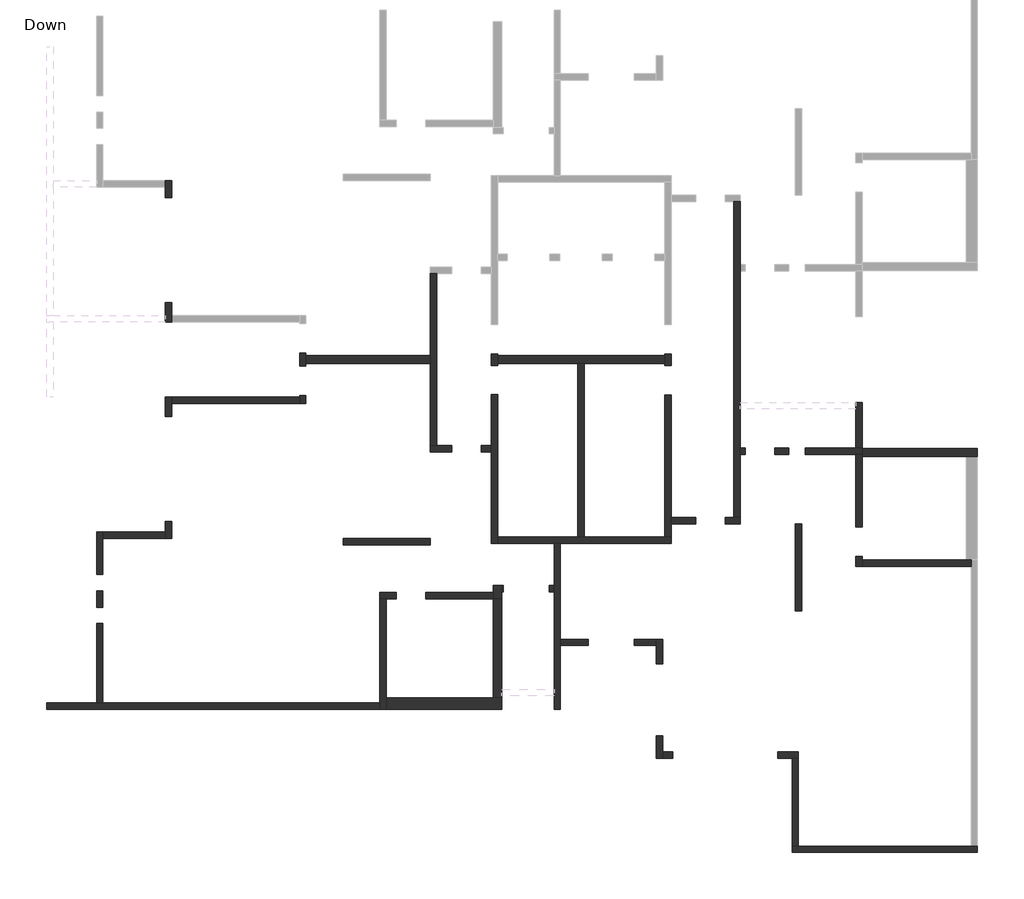
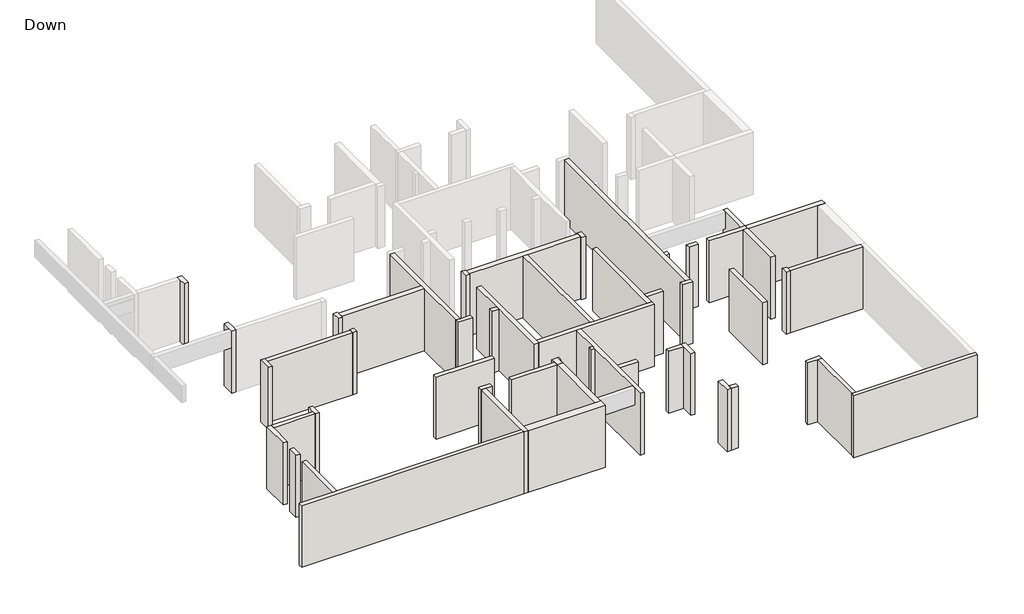
# One storey, part 1 of 2: 53 walls.
# Revit data of these elements (continued)
# Element 21 (IfcWall, "19") (continued)
#   SOFiSTiK_EdgeZones = "W41"
#   SOFiSTiK_AMG_Comments = "Too Short /"
#   Top Offset = 0 cm
#   Base Offset = 0 cm
#   wall height = 300 cm
#   SOFiSTiK_AMG_Scheduled = yes
#   SOFiSTiK_AMG_Adjusted = yes
#   Phase Created = New Construction
#   Base Constraint = Down
#   Top Constraint = Typical Floor
#   Materials on its faces: "Concrete"
# Element 22 (IfcWall, "19")
#   Comments = ""
#   Mark = "W42"
#   SOFiSTiK_EdgeZones = "W42"
#   SOFiSTiK_AMG_Comments = ""
#   Top Offset = 0 cm
#   Base Offset = 0 cm
#   wall height = 300 cm
#   SOFiSTiK_AMG_Scheduled = yes
#   SOFiSTiK_AMG_Adjusted = yes
#   Phase Created = New Construction
#   Base Constraint = Down
#   Top Constraint = Typical Floor
#   Materials on its faces: "Concrete"
# Element 23 (IfcWall, "20")
#   Comments = ""
#   Mark = "W59"
#   SOFiSTiK_EdgeZones = "W59"
#   SOFiSTiK_AMG_Comments = ""
#   Top Offset = 0 cm
#   Base Offset = 0 cm
#   wall height = 300 cm
#   SOFiSTiK_AMG_Scheduled = yes
#   SOFiSTiK_AMG_Adjusted = yes
#   Phase Created = New Construction
#   Base Constraint = Down
#   Top Constraint = Typical Floor
#   Materials on its faces: "Concrete"
# Element 24 (IfcWall, "20")
#   Comments = ""
#   Mark = "W60"
#   SOFiSTiK_EdgeZones = "W60"
#   SOFiSTiK_AMG_Comments = ""
#   Top Offset = 0 cm
#   Base Offset = 0 cm
#   wall height = 300 cm
#   SOFiSTiK_AMG_Scheduled = yes
#   SOFiSTiK_AMG_Adjusted = yes
#   Phase Created = New Construction
#   Base Constraint = Down
#   Top Constraint = Typical Floor
#   Materials on its faces: "Concrete"
# Element 25 (IfcWall, "20")
#   Comments = ""
#   Mark = "W75"
#   SOFiSTiK_EdgeZones = "W75"
#   SOFiSTiK_AMG_Comments = ""
#   Top Offset = 0 cm
#   Base Offset = 0 cm
#   wall height = 300 cm
#   SOFiSTiK_AMG_Scheduled = yes
#   SOFiSTiK_AMG_Adjusted = yes
#   Phase Created = New Construction
#   Base Constraint = Down
#   Top Constraint = Typical Floor
#   Materials on its faces: "Concrete"
# Element 26 (IfcWall, "20")
#   Comments = ""
#   Mark = "W76"
#   SOFiSTiK_EdgeZones = "W76"
#   SOFiSTiK_AMG_Comments = ""
#   Top Offset = 0 cm
#   Base Offset = 0 cm
#   wall height = 300 cm
#   SOFiSTiK_AMG_Scheduled = yes
#   SOFiSTiK_AMG_Adjusted = yes
#   Phase Created = New Construction
#   Base Constraint = Down
#   Top Constraint = Typical Floor
#   Materials on its faces: "Concrete"
# Element 27 (IfcWall, "20")
#   Comments = ""
#   Mark = "W77"
#   SOFiSTiK_EdgeZones = "W77"
#   SOFiSTiK_AMG_Comments = ""
#   Top Offset = 0 cm
#   Base Offset = 0 cm
#   wall height = 300 cm
#   SOFiSTiK_AMG_Scheduled = yes
#   SOFiSTiK_AMG_Adjusted = yes
#   Phase Created = New Construction
#   Base Constraint = Down
#   Top Constraint = Typical Floor
#   Materials on its faces: "Concrete"
# Element 28 (IfcWall, "20")
#   Comments = ""
#   Mark = "W78"
#   SOFiSTiK_EdgeZones = "W78"
#   SOFiSTiK_AMG_Comments = ""
#   Top Offset = 0 cm
#   Base Offset = 0 cm
#   wall height = 300 cm
#   SOFiSTiK_AMG_Scheduled = yes
#   SOFiSTiK_AMG_Adjusted = yes
#   Phase Created = New Construction
#   Base Constraint = Down
#   Top Constraint = Typical Floor
#   Materials on its faces: "Concrete"
# Element 29 (IfcWall, "20")
#   Comments = ""
#   Mark = "W79"
#   SOFiSTiK_EdgeZones = "W79"
#   SOFiSTiK_AMG_Comments = ""
#   Top Offset = 0 cm
#   Base Offset = 0 cm
#   wall height = 300 cm
#   SOFiSTiK_AMG_Scheduled = yes
#   SOFiSTiK_AMG_Adjusted = yes
#   Phase Created = New Construction
#   Base Constraint = Down
#   Top Constraint = Typical Floor
#   Materials on its faces: "Concrete"
# Element 30 (IfcWall, "20")
#   Comments = ""
#   Mark = "W80"
#   SOFiSTiK_EdgeZones = "W80"
#   SOFiSTiK_AMG_Comments = ""
#   Top Offset = 0 cm
#   Base Offset = 0 cm
#   wall height = 300 cm
#   SOFiSTiK_AMG_Scheduled = yes
#   SOFiSTiK_AMG_Adjusted = yes
#   Phase Created = New Construction
#   Base Constraint = Down
#   Top Constraint = Typical Floor
#   Materials on its faces: "Concrete"
# Element 31 (IfcWall, "20")
#   Comments = ""
#   Mark = "W81"
#   SOFiSTiK_EdgeZones = "W81"
#   SOFiSTiK_AMG_Comments = ""
#   Top Offset = 0 cm
#   Base Offset = 0 cm
#   wall height = 300 cm
#   SOFiSTiK_AMG_Scheduled = yes
#   SOFiSTiK_AMG_Adjusted = yes
#   Phase Created = New Construction
#   Base Constraint = Down
#   Top Constraint = Typical Floor
#   Materials on its faces: "Concrete"
# Element 32 (IfcWall, "20")
#   Comments = ""
#   Mark = "W82"
#   SOFiSTiK_EdgeZones = "W82"
#   SOFiSTiK_AMG_Comments = ""
#   Top Offset = 0 cm
#   Base Offset = 0 cm
#   wall height = 300 cm
#   SOFiSTiK_AMG_Scheduled = yes
#   SOFiSTiK_AMG_Adjusted = yes
#   Phase Created = New Construction
#   Base Constraint = Down
#   Top Constraint = Typical Floor
#   Materials on its faces: "Concrete"
# Element 33 (IfcWall, "20")
#   Comments = ""
#   Mark = "W83"
#   SOFiSTiK_EdgeZones = "W83"
#   SOFiSTiK_AMG_Comments = ""
#   Top Offset = 0 cm
#   Base Offset = 0 cm
#   wall height = 300 cm
#   SOFiSTiK_AMG_Scheduled = yes
#   SOFiSTiK_AMG_Adjusted = yes
#   Phase Created = New Construction
#   Base Constraint = Down
#   Top Constraint = Typical Floor
#   Materials on its faces: "Concrete"
# Element 34 (IfcWall, "20")
#   Comments = ""
#   Mark = "W84"
#   SOFiSTiK_EdgeZones = "W84"
#   SOFiSTiK_AMG_Comments = ""
#   Top Offset = 0 cm
#   Base Offset = 0 cm
#   wall height = 300 cm
#   SOFiSTiK_AMG_Scheduled = yes
#   SOFiSTiK_AMG_Adjusted = yes
#   Phase Created = New Construction
#   Base Constraint = Down
#   Top Constraint = Typical Floor
#   Materials on its faces: "Concrete"
# Element 35 (IfcWall, "20")
#   Comments = ""
#   Mark = "W85"
#   SOFiSTiK_EdgeZones = "W85"
#   SOFiSTiK_AMG_Comments = ""
#   Top Offset = 0 cm
#   Base Offset = 0 cm
#   wall height = 300 cm
#   SOFiSTiK_AMG_Scheduled = yes
#   SOFiSTiK_AMG_Adjusted = yes
#   Phase Created = New Construction
#   Base Constraint = Down
#   Top Constraint = Typical Floor
#   Materials on its faces: "Concrete"
# Element 36 (IfcWall, "20")
#   Comments = ""
#   Mark = "W87"
#   SOFiSTiK_EdgeZones = "W87"
#   SOFiSTiK_AMG_Comments = ""
#   Top Offset = 0 cm
#   Base Offset = 0 cm
#   wall height = 300 cm
#   SOFiSTiK_AMG_Scheduled = yes
#   SOFiSTiK_AMG_Adjusted = yes
#   Phase Created = New Construction
#   Base Constraint = Down
#   Top Constraint = Typical Floor
#   Materials on its faces: "Concrete"
# Element 37 (IfcWall, "20")
#   Comments = ""
#   Mark = "W88"
#   SOFiSTiK_EdgeZones = "W88"
#   SOFiSTiK_AMG_Comments = ""
#   Top Offset = 0 cm
#   Base Offset = 0 cm
#   wall height = 300 cm
#   SOFiSTiK_AMG_Scheduled = yes
#   SOFiSTiK_AMG_Adjusted = yes
#   Phase Created = New Construction
#   Base Constraint = Down
#   Top Constraint = Typical Floor
#   Materials on its faces: "Concrete"
# Element 38 (IfcWall, "20")
#   Comments = ""
#   Mark = "W89"
#   SOFiSTiK_EdgeZones = "W89"
#   SOFiSTiK_AMG_Comments = ""
#   Top Offset = 0 cm
#   Base Offset = 0 cm
#   wall height = 300 cm
#   SOFiSTiK_AMG_Scheduled = yes
#   SOFiSTiK_AMG_Adjusted = yes
#   Phase Created = New Construction
#   Base Constraint = Down
#   Top Constraint = Typical Floor
#   Materials on its faces: "Concrete"
# Element 39 (IfcWall, "20")
#   Comments = ""
#   Mark = "W90"
#   SOFiSTiK_EdgeZones = "W90"
#   SOFiSTiK_AMG_Comments = ""
#   Top Offset = 0 cm
#   Base Offset = 0 cm
#   wall height = 300 cm
#   SOFiSTiK_AMG_Scheduled = yes
#   SOFiSTiK_AMG_Adjusted = yes
#   Phase Created = New Construction
#   Base Constraint = Down
#   Top Constraint = Typical Floor
#   Materials on its faces: "Concrete"
# Element 40 (IfcWall, "20")
#   Comments = ""
#   Mark = "W92"
#   SOFiSTiK_EdgeZones = "W92"
#   SOFiSTiK_AMG_Comments = "Too Short /"
#   Top Offset = 0 cm
#   Base Offset = 0 cm
#   wall height = 300 cm
#   SOFiSTiK_AMG_Scheduled = yes
#   SOFiSTiK_AMG_Adjusted = yes
#   Phase Created = New Construction
#   Base Constraint = Down
#   Top Constraint = Typical Floor
#   Materials on its faces: "Concrete"
# Element 41 (IfcWall, "20")
#   Comments = ""
#   Mark = "W93"
#   SOFiSTiK_EdgeZones = "W93"
#   SOFiSTiK_AMG_Comments = ""
#   Top Offset = 0 cm
#   Base Offset = 0 cm
#   wall height = 300 cm
#   SOFiSTiK_AMG_Scheduled = yes
#   SOFiSTiK_AMG_Adjusted = yes
#   Phase Created = New Construction
#   Base Constraint = Down
#   Top Constraint = Typical Floor
#   Materials on its faces: "Concrete"
# Element 42 (IfcWall, "20")
#   Comments = ""
#   Mark = "W94"
#   SOFiSTiK_EdgeZones = "W94"
#   SOFiSTiK_AMG_Comments = ""
#   Top Offset = 0 cm
#   Base Offset = 0 cm
#   wall height = 300 cm
#   SOFiSTiK_AMG_Scheduled = yes
#   SOFiSTiK_AMG_Adjusted = yes
#   Phase Created = New Construction
#   Base Constraint = Down
#   Top Constraint = Typical Floor
#   Materials on its faces: "Concrete"
# Element 43 (IfcWall, "20")
#   Comments = ""
#   Mark = "W95"
#   SOFiSTiK_EdgeZones = "W95"
#   SOFiSTiK_AMG_Comments = ""
#   Top Offset = 0 cm
#   Base Offset = 0 cm
#   wall height = 300 cm
#   SOFiSTiK_AMG_Scheduled = yes
#   SOFiSTiK_AMG_Adjusted = yes
#   Phase Created = New Construction
#   Base Constraint = Down
#   Top Constraint = Typical Floor
#   Materials on its faces: "Concrete"
# Element 44 (IfcWall, "20")
#   Comments = ""
#   Mark = "W96"
#   SOFiSTiK_EdgeZones = "W96"
#   SOFiSTiK_AMG_Comments = ""
#   Top Offset = 0 cm
#   Base Offset = 0 cm
#   wall height = 300 cm
#   SOFiSTiK_AMG_Scheduled = yes
#   SOFiSTiK_AMG_Adjusted = yes
#   Phase Created = New Construction
#   Base Constraint = Down
#   Top Constraint = Typical Floor
#   Materials on its faces: "Concrete"
# Element 45 (IfcWall, "20")
#   Comments = ""
#   Mark = "W97"
#   SOFiSTiK_EdgeZones = "W97"
#   SOFiSTiK_AMG_Comments = ""
#   Top Offset = 0 cm
#   Base Offset = 0 cm
#   wall height = 300 cm
#   SOFiSTiK_AMG_Scheduled = yes
#   SOFiSTiK_AMG_Adjusted = yes
#   Phase Created = New Construction
#   Base Constraint = Down
#   Top Constraint = Typical Floor
#   Materials on its faces: "Concrete"
# Element 46 (IfcWall, "20")
#   Comments = ""
#   Mark = "W98"
#   SOFiSTiK_EdgeZones = "W98"
#   SOFiSTiK_AMG_Comments = ""
#   Top Offset = 0 cm
#   Base Offset = 0 cm
#   wall height = 300 cm
#   SOFiSTiK_AMG_Scheduled = yes
#   SOFiSTiK_AMG_Adjusted = yes
#   Phase Created = New Construction
#   Base Constraint = Down
#   Top Constraint = Typical Floor
#   Materials on its faces: "Concrete"
# Element 47 (IfcWall, "20")
#   Comments = ""
#   Mark = "W99"
#   SOFiSTiK_EdgeZones = "W99"
#   SOFiSTiK_AMG_Comments = ""
#   Top Offset = 0 cm
#   Base Offset = 0 cm
#   wall height = 300 cm
#   SOFiSTiK_AMG_Scheduled = yes
#   SOFiSTiK_AMG_Adjusted = yes
#   Phase Created = New Construction
#   Base Constraint = Down
#   Top Constraint = Typical Floor
#   Materials on its faces: "Concrete"
# Element 48 (IfcWall, "25")
#   Comments = ""
#   Mark = "W100"
#   SOFiSTiK_EdgeZones = "W100"
#   SOFiSTiK_AMG_Comments = ""
#   Top Offset = 0 cm
#   Base Offset = 0 cm
#   wall height = 300 cm
#   SOFiSTiK_AMG_Scheduled = yes
#   SOFiSTiK_AMG_Adjusted = yes
#   Phase Created = New Construction
#   Base Constraint = Down
#   Top Constraint = Typical Floor
#   Materials on its faces: "Concrete"
# Element 49 (IfcWall, "25")
#   Comments = ""
#   Mark = "W103"
#   SOFiSTiK_EdgeZones = "W103"
#   SOFiSTiK_AMG_Comments = ""
#   Top Offset = 0 cm
#   Base Offset = 0 cm
#   wall height = 300 cm
#   SOFiSTiK_AMG_Scheduled = yes
#   SOFiSTiK_AMG_Adjusted = yes
#   Phase Created = New Construction
#   Base Constraint = Down
#   Top Constraint = Typical Floor
#   Materials on its faces: "Concrete"
# Element 50 (IfcWall, "25")
#   Comments = ""
#   Mark = "W105"
#   SOFiSTiK_EdgeZones = "W105"
#   SOFiSTiK_AMG_Comments = ""
#   Top Offset = 0 cm
#   Base Offset = 0 cm
#   wall height = 300 cm
#   SOFiSTiK_AMG_Scheduled = yes
#   SOFiSTiK_AMG_Adjusted = yes
#   Phase Created = New Construction
#   Base Constraint = Down
#   Top Constraint = Typical Floor
#   Materials on its faces: "Concrete"
# Element 51 (IfcWall, "25")
#   Comments = ""
#   Mark = "W106"
#   SOFiSTiK_EdgeZones = "W106"
#   SOFiSTiK_AMG_Comments = ""
#   Top Offset = 0 cm
#   Base Offset = 0 cm
#   wall height = 300 cm
#   SOFiSTiK_AMG_Scheduled = yes
#   SOFiSTiK_AMG_Adjusted = yes
#   Phase Created = New Construction
#   Base Constraint = Down
#   Top Constraint = Typical Floor
#   Materials on its faces: "Concrete"
# Element 52 (IfcWall, "25")
#   Comments = ""
#   Mark = "W107"
#   SOFiSTiK_EdgeZones = "W107"
#   SOFiSTiK_AMG_Comments = ""
#   Top Offset = 0 cm
#   Base Offset = 0 cm
#   wall height = 300 cm
#   SOFiSTiK_AMG_Scheduled = yes
#   SOFiSTiK_AMG_Adjusted = yes
#   Phase Created = New Construction
#   Base Constraint = Down
#   Top Constraint = Typical Floor
#   Materials on its faces: "Concrete"
# Element 53 (IfcWall, "35")
#   Comments = ""
#   Mark = "W110"
#   SOFiSTiK_EdgeZones = "W110"
#   SOFiSTiK_AMG_Comments = ""
#   Top Offset = 0 cm
#   Base Offset = 0 cm
#   wall height = 300 cm
#   SOFiSTiK_AMG_Scheduled = yes
#   SOFiSTiK_AMG_Adjusted = yes
#   Phase Created = New Construction
#   Base Constraint = Down
#   Top Constraint = Typical Floor
#   Materials on its faces: "Concrete"
# Materials
#   "Concrete": class "Concrete", colour RGB 192 192 192, transparency 0, Keynote = "01000", Description = "Cast-in-place concrete", Cost = 0
